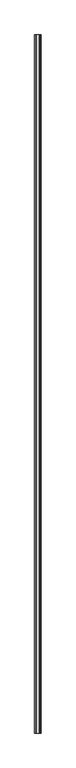
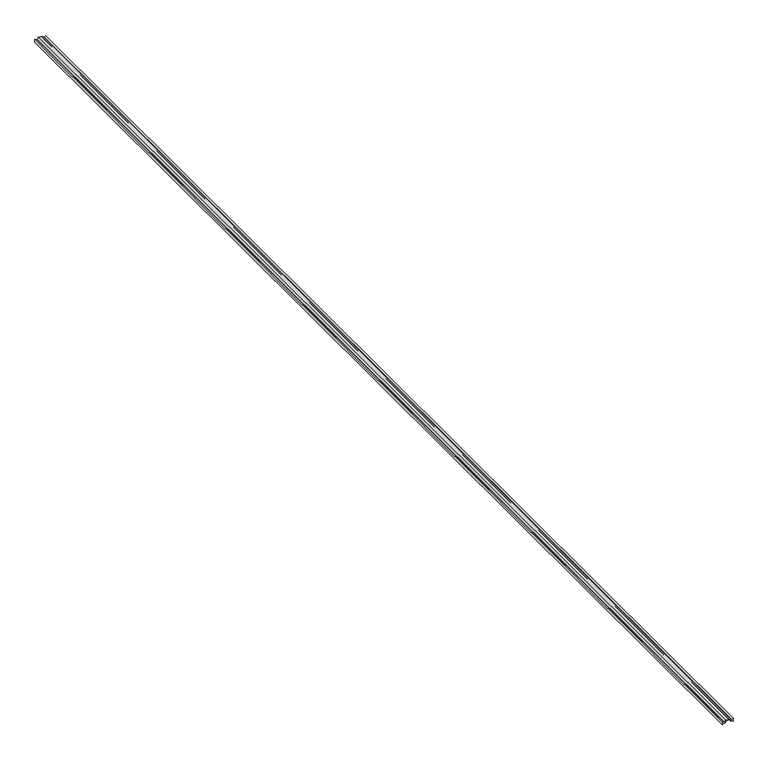
"""IFC4 building model written with IfcOpenShell, lengths in millimetres: proxy geometry, Door frame10:Door frame010:296308 : Door frame10:Door frame010:296308."""

import ifcopenshell
import ifcopenshell.guid

model = None  # the IFC model being written
_history = None  # IfcOwnerHistory: only IFC2X3 demands one
_inside = {}  # id of a spatial element -> (the spatial element, [elements in it])
_under = {}  # id of a project, library or spatial element -> (it, [spatial elements below it])
_declared = {}  # id of a project -> (the project, [libraries it declares])
_typed = {}  # id of a type object -> (the type object, [elements of that type])
_made_of = {}  # id of a material, layer set ... -> (it, [elements and type objects made of it])


def new_model(schema):
    """Start an empty IFC model of exactly this schema.

    Asked for "IFC4X3", IfcOpenShell would pick the latest addendum, in which some entities
    have other attributes; the version numbers below select the first issue.
    IFC2X3 requires an IfcOwnerHistory on every rooted entity: one is made here for all.
    """
    global model, _history
    if schema == "IFC4X3":
        model = ifcopenshell.file(schema_version=(4, 3, 0, 0))
    else:
        model = ifcopenshell.file(schema=schema)
    _inside.clear()
    _under.clear()
    _declared.clear()
    _typed.clear()
    _made_of.clear()
    _history = None
    if model.schema == "IFC2X3":
        org = make("IfcOrganization", Name="unknown")
        user = make(
            "IfcPersonAndOrganization",
            ThePerson=make("IfcPerson", FamilyName="unknown"),
            TheOrganization=org,
        )
        app = make(
            "IfcApplication",
            ApplicationDeveloper=org,
            Version="unknown",
            ApplicationFullName="unknown",
            ApplicationIdentifier="unknown",
        )
        _history = make(
            "IfcOwnerHistory",
            OwningUser=user,
            OwningApplication=app,
            ChangeAction="ADDED",
            CreationDate=0,
        )
    return model


def make(cls, **values):
    """One entity of the class cls with the attributes given. An attribute that is None is left unset."""
    return model.create_entity(
        cls, **{name: value for name, value in values.items() if value is not None}
    )


def rooted(cls, **values):
    """An entity with a GlobalId (a new one), such as an element, a storey or a relation."""
    return make(cls, GlobalId=ifcopenshell.guid.new(), OwnerHistory=_history, **values)


def si_unit(unit_type, name, prefix=None):
    """IfcSIUnit, for example si_unit("LENGTHUNIT", "METRE", prefix="MILLI")."""
    return make("IfcSIUnit", UnitType=unit_type, Prefix=prefix, Name=name)


def assignment(units):
    """IfcUnitAssignment: the units of a project."""
    return None if units is None else make("IfcUnitAssignment", Units=units)


def point(xyz):
    """IfcCartesianPoint."""
    return None if xyz is None else make("IfcCartesianPoint", Coordinates=xyz)


def direction(xyz):
    """IfcDirection."""
    return None if xyz is None else make("IfcDirection", DirectionRatios=xyz)


def frame(location, z_axis=None, x_axis=None):
    """IfcAxis2Placement3D, a coordinate frame: its origin and axes. An axis left out is left unset."""
    return make(
        "IfcAxis2Placement3D",
        Location=point(location),
        Axis=direction(z_axis),
        RefDirection=direction(x_axis),
    )


def origin():
    """The frame at (0, 0, 0) with its axes left unset."""
    return frame((0.0, 0.0, 0.0))


def place(relative_to, where):
    """IfcLocalPlacement: puts the frame where relative to a parent placement (None: the world)."""
    return make(
        "IfcLocalPlacement", PlacementRelTo=relative_to, RelativePlacement=where
    )


def context(
    kind, dimensions, precision=None, world=None, true_north=None, identifier=None
):
    """IfcGeometricRepresentationContext, for example the 3D "Model" context."""
    return make(
        "IfcGeometricRepresentationContext",
        ContextIdentifier=identifier,
        ContextType=kind,
        CoordinateSpaceDimension=dimensions,
        Precision=precision,
        WorldCoordinateSystem=world,
        TrueNorth=true_north,
    )


def project(units=None, contexts=None):
    """IfcProject with its units and contexts."""
    return rooted(
        "IfcProject",
        Name="project",
        RepresentationContexts=contexts,
        UnitsInContext=assignment(units),
    )


def spatial(cls, under=None, at=None, **own):
    """A site, building, storey or space (cls), placed at a placement, below another one or the project."""
    s = rooted(cls, ObjectPlacement=at, **own)
    if under is not None:
        _under.setdefault(under.id(), (under, []))[1].append(s)
    return s


def polyline(points):
    """IfcPolyline through the points."""
    return make("IfcPolyline", Points=[point(p) for p in points])


def outline(outer, holes=None, kind="AREA"):
    """IfcArbitraryClosedProfileDef: a profile drawn as a closed curve; with holes, ...WithVoids."""
    if holes is None:
        return make("IfcArbitraryClosedProfileDef", ProfileType=kind, OuterCurve=outer)
    return make(
        "IfcArbitraryProfileDefWithVoids",
        ProfileType=kind,
        OuterCurve=outer,
        InnerCurves=holes,
    )


def extrude(swept, where, along, depth):
    """IfcExtrudedAreaSolid: the profile swept, set in the frame where, extruded along a direction by depth."""
    return make(
        "IfcExtrudedAreaSolid",
        SweptArea=swept,
        Position=where,
        ExtrudedDirection=direction(along),
        Depth=depth,
    )


def shape(context_of_items, identifier, shape_type, items):
    """IfcShapeRepresentation: the items that make up one representation, for example the "Body"."""
    return make(
        "IfcShapeRepresentation",
        ContextOfItems=context_of_items,
        RepresentationIdentifier=identifier,
        RepresentationType=shape_type,
        Items=items,
    )


def source(mapping_origin, context_of_items, identifier, shape_type, items):
    """IfcRepresentationMap: a shape defined once, which mapped items show again and again."""
    return make(
        "IfcRepresentationMap",
        MappingOrigin=mapping_origin,
        MappedRepresentation=shape(context_of_items, identifier, shape_type, items),
    )


def transform(
    local_origin,
    x_axis=None,
    y_axis=None,
    z_axis=None,
    scale=None,
    scale2=None,
    scale3=None,
    uniform=True,
):
    """IfcCartesianTransformationOperator3D, or its non-uniform kind. x_axis, y_axis, z_axis: its Axis1, 2, 3."""
    if uniform:
        return make(
            "IfcCartesianTransformationOperator3D",
            Axis1=direction(x_axis),
            Axis2=direction(y_axis),
            LocalOrigin=point(local_origin),
            Scale=scale,
            Axis3=direction(z_axis),
        )
    return make(
        "IfcCartesianTransformationOperator3DnonUniform",
        Axis1=direction(x_axis),
        Axis2=direction(y_axis),
        LocalOrigin=point(local_origin),
        Scale=scale,
        Axis3=direction(z_axis),
        Scale2=scale2,
        Scale3=scale3,
    )


def mapped(mapping_source, mapping_target):
    """IfcMappedItem: shows the shape of a source again, moved by a transform."""
    return make(
        "IfcMappedItem", MappingSource=mapping_source, MappingTarget=mapping_target
    )


def made_of(thing, what):
    """Note that an element or type object is made of a material, layer set ...; save() writes the relation."""
    if what is not None:
        _made_of.setdefault(what.id(), (what, []))[1].append(thing)
    return thing


def element(
    cls,
    number,
    at=None,
    inside=None,
    cuts=None,
    type_object=None,
    material=None,
    context=None,
    identifier="Body",
    shape_type=None,
    held_by="IfcProductDefinitionShape",
    body=None,
    shapes=None,
    **own,
):
    """One element of the class cls, such as IfcWall. Its Tag is "e" and its number.

    at: its placement. inside: the storey or other place that contains it. cuts: it is an
    opening in that element (IfcRelVoidsElement). A single representation is given by context,
    identifier, shape_type and body (its items); several are given by shapes. held_by: the class
    of the entity that holds the representations. save() writes the other relations.
    """
    e = rooted(cls, Tag="e%d" % number, ObjectPlacement=at, **own)
    if body is not None:
        shapes = [shape(context, identifier, shape_type, body)]
    if shapes is not None:
        e.Representation = make(held_by, Representations=shapes)
    if inside is not None:
        _inside.setdefault(inside.id(), (inside, []))[1].append(e)
    if cuts is not None:
        rooted(
            "IfcRelVoidsElement", RelatingBuildingElement=cuts, RelatedOpeningElement=e
        )
    if type_object is not None:
        _typed.setdefault(type_object.id(), (type_object, []))[1].append(e)
    return made_of(e, material)


def aggregate(whole, parts):
    """IfcRelAggregates: a whole, such as a stair, and the parts it consists of."""
    return rooted("IfcRelAggregates", RelatingObject=whole, RelatedObjects=parts)


def save(model, path):
    """Write the relations noted so far, then the file.

    IfcRelAggregates (storeys below a building ...), IfcRelContainedInSpatialStructure (elements
    in a storey), IfcRelDefinesByType, IfcRelAssociatesMaterial and IfcRelDeclares: one each for
    every whole, place, type object, material and project.
    """
    for whole, parts in _under.values():
        aggregate(whole, parts)
    for where, things in _inside.values():
        rooted(
            "IfcRelContainedInSpatialStructure",
            RelatedElements=things,
            RelatingStructure=where,
        )
    for kind, things in _typed.values():
        rooted("IfcRelDefinesByType", RelatedObjects=things, RelatingType=kind)
    for what, things in _made_of.values():
        rooted("IfcRelAssociatesMaterial", RelatedObjects=things, RelatingMaterial=what)
    for by, libraries in _declared.values():
        rooted("IfcRelDeclares", RelatingContext=by, RelatedDefinitions=libraries)
    model.write(path)


def generic_models_afd02588(model_context):
    return source(origin(), model_context, "Body", "SweptSolid", [
        extrude(outline(polyline([(36661.0991325, 20312.8043864), (36662.6580816, 20315.5045655), (36662.6580816, 20317.1510686), (36665.8580816, 20319.3917327), (36665.8580816, 20324.7404765), (36662.6580816, 20326.9811406), (36662.6580816, 20328.6276436), (36661.1287449, 20331.2765325), (36665.9874184, 20331.2765325), (36664.4580816, 20328.6276436), (36664.4580816, 20327.6740064), (36667.4580816, 20325.5733837), (36667.4580816, 20318.5588254), (36664.4580816, 20316.4582028), (36664.4580816, 20315.5045655), (36666.0170308, 20312.8043864), (36661.0991325, 20312.8043864)])), frame((0.0, -774.5581156, 0.0), z_axis=(0.0, 1.0, 0.0), x_axis=(0.0, 0.0, 1.0)), (0.0, 0.0, 1.0), 1999.85),
    ])


if __name__ == "__main__":
    model = new_model("IFC4")
    model_context = context("Model", 3, world=origin())
    ifc_project = project(units=[si_unit("LENGTHUNIT", "METRE", prefix="MILLI")], contexts=[model_context])
    site = spatial("IfcSite", under=ifc_project)
    building = spatial("IfcBuilding", under=site)
    placement = place(None, origin())
    generic_models_shape = generic_models_afd02588(model_context)
    element("IfcBuildingElementProxy", 1, Name="Door frame10:Door frame010:296308 : Door frame10:Door frame010:296308", ObjectType="Door frame10:Door frame010:296308 : Door frame10:Door frame010:296308", at=placement, inside=building, context=model_context, shape_type="MappedRepresentation", body=[
        mapped(generic_models_shape, transform((0.0, 0.0, 0.0), x_axis=(1.0, 0.0, 0.0), y_axis=(0.0, 1.0, 0.0), z_axis=(0.0, 0.0, 1.0))),
    ])
    save(model, "model.ifc")

# Revit data of these elements
# Type "Door frame10:Door frame010:296308 : Door frame10:Door frame010:296308"
#   NameOverride = "Door frame10:Door frame010:296308"
#   ObjectTypeOverride = "Door frame10:Door frame010"
#   Reference = "Door frame010"
#   Category = "Generic Models"
#   Tag = "296308"
# Element 1 (IfcBuildingElementProxy, "Door frame10:Door frame010:296308 : Door frame10:Door frame010:296308")
#   Materials on its faces: "FLEETWOOD SERIES T-3200 SINGLE SWING DOOR FRAME"
# Materials
#   "FLEETWOOD SERIES T-3200 SINGLE SWING DOOR FRAME": class "Unassigned", colour RGB 128 128 128, transparency 0, Cost = 0
